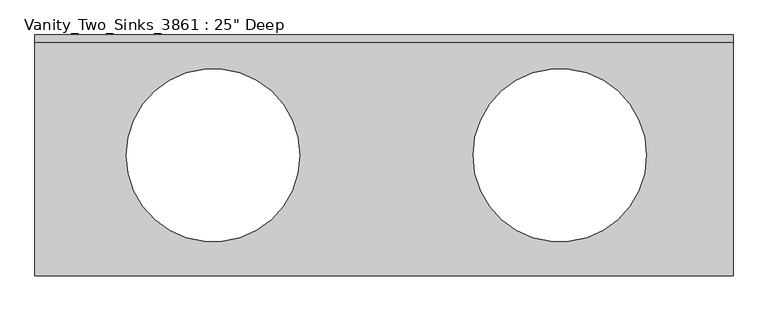
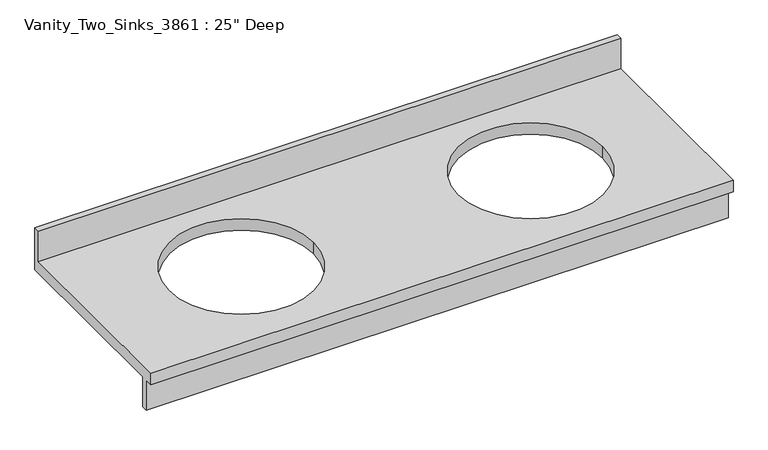
"""IFC4 building model written with IfcOpenShell, lengths in millimetres: furniture geometry."""

import ifcopenshell
import ifcopenshell.guid

model = None  # the IFC model being written
_history = None  # IfcOwnerHistory: only IFC2X3 demands one
_inside = {}  # id of a spatial element -> (the spatial element, [elements in it])
_under = {}  # id of a project, library or spatial element -> (it, [spatial elements below it])
_declared = {}  # id of a project -> (the project, [libraries it declares])
_typed = {}  # id of a type object -> (the type object, [elements of that type])
_made_of = {}  # id of a material, layer set ... -> (it, [elements and type objects made of it])


def new_model(schema):
    """Start an empty IFC model of exactly this schema.

    Asked for "IFC4X3", IfcOpenShell would pick the latest addendum, in which some entities
    have other attributes; the version numbers below select the first issue.
    IFC2X3 requires an IfcOwnerHistory on every rooted entity: one is made here for all.
    """
    global model, _history
    if schema == "IFC4X3":
        model = ifcopenshell.file(schema_version=(4, 3, 0, 0))
    else:
        model = ifcopenshell.file(schema=schema)
    _inside.clear()
    _under.clear()
    _declared.clear()
    _typed.clear()
    _made_of.clear()
    _history = None
    if model.schema == "IFC2X3":
        org = make("IfcOrganization", Name="unknown")
        user = make(
            "IfcPersonAndOrganization",
            ThePerson=make("IfcPerson", FamilyName="unknown"),
            TheOrganization=org,
        )
        app = make(
            "IfcApplication",
            ApplicationDeveloper=org,
            Version="unknown",
            ApplicationFullName="unknown",
            ApplicationIdentifier="unknown",
        )
        _history = make(
            "IfcOwnerHistory",
            OwningUser=user,
            OwningApplication=app,
            ChangeAction="ADDED",
            CreationDate=0,
        )
    return model


def make(cls, **values):
    """One entity of the class cls with the attributes given. An attribute that is None is left unset."""
    return model.create_entity(
        cls, **{name: value for name, value in values.items() if value is not None}
    )


def rooted(cls, **values):
    """An entity with a GlobalId (a new one), such as an element, a storey or a relation."""
    return make(cls, GlobalId=ifcopenshell.guid.new(), OwnerHistory=_history, **values)


def si_unit(unit_type, name, prefix=None):
    """IfcSIUnit, for example si_unit("LENGTHUNIT", "METRE", prefix="MILLI")."""
    return make("IfcSIUnit", UnitType=unit_type, Prefix=prefix, Name=name)


def assignment(units):
    """IfcUnitAssignment: the units of a project."""
    return None if units is None else make("IfcUnitAssignment", Units=units)


def point(xyz):
    """IfcCartesianPoint."""
    return None if xyz is None else make("IfcCartesianPoint", Coordinates=xyz)


def direction(xyz):
    """IfcDirection."""
    return None if xyz is None else make("IfcDirection", DirectionRatios=xyz)


def frame(location, z_axis=None, x_axis=None):
    """IfcAxis2Placement3D, a coordinate frame: its origin and axes. An axis left out is left unset."""
    return make(
        "IfcAxis2Placement3D",
        Location=point(location),
        Axis=direction(z_axis),
        RefDirection=direction(x_axis),
    )


def origin():
    """The frame at (0, 0, 0) with its axes left unset."""
    return frame((0.0, 0.0, 0.0))


def place(relative_to, where):
    """IfcLocalPlacement: puts the frame where relative to a parent placement (None: the world)."""
    return make(
        "IfcLocalPlacement", PlacementRelTo=relative_to, RelativePlacement=where
    )


def context(
    kind, dimensions, precision=None, world=None, true_north=None, identifier=None
):
    """IfcGeometricRepresentationContext, for example the 3D "Model" context."""
    return make(
        "IfcGeometricRepresentationContext",
        ContextIdentifier=identifier,
        ContextType=kind,
        CoordinateSpaceDimension=dimensions,
        Precision=precision,
        WorldCoordinateSystem=world,
        TrueNorth=true_north,
    )


def project(units=None, contexts=None):
    """IfcProject with its units and contexts."""
    return rooted(
        "IfcProject",
        Name="project",
        RepresentationContexts=contexts,
        UnitsInContext=assignment(units),
    )


def spatial(cls, under=None, at=None, **own):
    """A site, building, storey or space (cls), placed at a placement, below another one or the project."""
    s = rooted(cls, ObjectPlacement=at, **own)
    if under is not None:
        _under.setdefault(under.id(), (under, []))[1].append(s)
    return s


def polyline(points):
    """IfcPolyline through the points."""
    return make("IfcPolyline", Points=[point(p) for p in points])


def circle_curve(where, radius):
    """IfcCircle in the frame where."""
    return make("IfcCircle", Position=where, Radius=radius)


def shape(context_of_items, identifier, shape_type, items):
    """IfcShapeRepresentation: the items that make up one representation, for example the "Body"."""
    return make(
        "IfcShapeRepresentation",
        ContextOfItems=context_of_items,
        RepresentationIdentifier=identifier,
        RepresentationType=shape_type,
        Items=items,
    )


def source(mapping_origin, context_of_items, identifier, shape_type, items):
    """IfcRepresentationMap: a shape defined once, which mapped items show again and again."""
    return make(
        "IfcRepresentationMap",
        MappingOrigin=mapping_origin,
        MappedRepresentation=shape(context_of_items, identifier, shape_type, items),
    )


def transform(
    local_origin,
    x_axis=None,
    y_axis=None,
    z_axis=None,
    scale=None,
    scale2=None,
    scale3=None,
    uniform=True,
):
    """IfcCartesianTransformationOperator3D, or its non-uniform kind. x_axis, y_axis, z_axis: its Axis1, 2, 3."""
    if uniform:
        return make(
            "IfcCartesianTransformationOperator3D",
            Axis1=direction(x_axis),
            Axis2=direction(y_axis),
            LocalOrigin=point(local_origin),
            Scale=scale,
            Axis3=direction(z_axis),
        )
    return make(
        "IfcCartesianTransformationOperator3DnonUniform",
        Axis1=direction(x_axis),
        Axis2=direction(y_axis),
        LocalOrigin=point(local_origin),
        Scale=scale,
        Axis3=direction(z_axis),
        Scale2=scale2,
        Scale3=scale3,
    )


def mapped(mapping_source, mapping_target):
    """IfcMappedItem: shows the shape of a source again, moved by a transform."""
    return make(
        "IfcMappedItem", MappingSource=mapping_source, MappingTarget=mapping_target
    )


def made_of(thing, what):
    """Note that an element or type object is made of a material, layer set ...; save() writes the relation."""
    if what is not None:
        _made_of.setdefault(what.id(), (what, []))[1].append(thing)
    return thing


def element(
    cls,
    number,
    at=None,
    inside=None,
    cuts=None,
    type_object=None,
    material=None,
    context=None,
    identifier="Body",
    shape_type=None,
    held_by="IfcProductDefinitionShape",
    body=None,
    shapes=None,
    **own,
):
    """One element of the class cls, such as IfcWall. Its Tag is "e" and its number.

    at: its placement. inside: the storey or other place that contains it. cuts: it is an
    opening in that element (IfcRelVoidsElement). A single representation is given by context,
    identifier, shape_type and body (its items); several are given by shapes. held_by: the class
    of the entity that holds the representations. save() writes the other relations.
    """
    e = rooted(cls, Tag="e%d" % number, ObjectPlacement=at, **own)
    if body is not None:
        shapes = [shape(context, identifier, shape_type, body)]
    if shapes is not None:
        e.Representation = make(held_by, Representations=shapes)
    if inside is not None:
        _inside.setdefault(inside.id(), (inside, []))[1].append(e)
    if cuts is not None:
        rooted(
            "IfcRelVoidsElement", RelatingBuildingElement=cuts, RelatedOpeningElement=e
        )
    if type_object is not None:
        _typed.setdefault(type_object.id(), (type_object, []))[1].append(e)
    return made_of(e, material)


def aggregate(whole, parts):
    """IfcRelAggregates: a whole, such as a stair, and the parts it consists of."""
    return rooted("IfcRelAggregates", RelatingObject=whole, RelatedObjects=parts)


def save(model, path):
    """Write the relations noted so far, then the file.

    IfcRelAggregates (storeys below a building ...), IfcRelContainedInSpatialStructure (elements
    in a storey), IfcRelDefinesByType, IfcRelAssociatesMaterial and IfcRelDeclares: one each for
    every whole, place, type object, material and project.
    """
    for whole, parts in _under.values():
        aggregate(whole, parts)
    for where, things in _inside.values():
        rooted(
            "IfcRelContainedInSpatialStructure",
            RelatedElements=things,
            RelatingStructure=where,
        )
    for kind, things in _typed.values():
        rooted("IfcRelDefinesByType", RelatedObjects=things, RelatingType=kind)
    for what, things in _made_of.values():
        rooted("IfcRelAssociatesMaterial", RelatedObjects=things, RelatingMaterial=what)
    for by, libraries in _declared.values():
        rooted("IfcRelDeclares", RelatingContext=by, RelatedDefinitions=libraries)
    model.write(path)


def plane_surface(at):
    """IfcPlane: the flat surface through the origin of the frame at, square to its z axis."""
    return make("IfcPlane", Position=at)


def revolved_surface(curve, axis_point, axis_direction):
    """IfcSurfaceOfRevolution: the curve turned about the line through axis_point along axis_direction."""
    return make(
        "IfcSurfaceOfRevolution",
        SweptCurve=make("IfcArbitraryOpenProfileDef", ProfileType="CURVE", Curve=curve),
        AxisPosition=make("IfcAxis1Placement", Location=point(axis_point), Axis=direction(axis_direction)),
    )


def advanced_brep(points, edges, surfaces, faces):
    """IfcAdvancedBrep: a solid bounded by faces that lie on surfaces and meet in shared edges.

    An edge is (start, end): straight between two places in points (the first is 0);
    or (start, end, curve); or (start, end, curve, False) where it runs against its curve.
    A face is (place in surfaces, loops), or (place, loops, False) where it looks against
    its surface's normal. A loop lists edges by number (the first is 1), with a minus sign
    where the edge is run from its end to its start. The first loop is the outer one.
    """
    corners = [point(p) for p in points]
    vertices = [make("IfcVertexPoint", VertexGeometry=c) for c in corners]
    made = []
    for start, end, *more in edges:
        made.append(
            make(
                "IfcEdgeCurve",
                EdgeStart=vertices[start],
                EdgeEnd=vertices[end],
                EdgeGeometry=more[0] if more else make("IfcPolyline", Points=[corners[start], corners[end]]),
                SameSense=more[1] if len(more) > 1 else True,
            )
        )
    hull = []
    for where, loops, *sense in faces:
        bounds = []
        for j, loop in enumerate(loops):
            ring = [make("IfcOrientedEdge", EdgeElement=made[abs(k) - 1], Orientation=k > 0) for k in loop]
            bounds.append(
                make(
                    "IfcFaceOuterBound" if j == 0 else "IfcFaceBound",
                    Bound=make("IfcEdgeLoop", EdgeList=ring),
                    Orientation=True,
                )
            )
        hull.append(make("IfcAdvancedFace", Bounds=bounds, FaceSurface=surfaces[where], SameSense=sense[0] if sense else True))
    return make("IfcAdvancedBrep", Outer=make("IfcClosedShell", CfsFaces=hull))


def furniture_801237fe(model_context):
    return source(origin(), model_context, "Body", "AdvancedBrep", [
        advanced_brep(
        [(-1327.4622951, -635.0, 863.6), (514.0377049, -635.0, 863.6), (514.0377049, -19.05, 863.6), (-1327.4622951, -19.05, 863.6), (285.4377049, -317.5, 863.6), (-171.7622951, -317.5, 863.6), (-628.9622951, -317.5, 863.6), (-1086.1622951, -317.5, 863.6), (514.0377049, -635.0, 825.5), (-1327.4622951, -635.0, 825.5), (-1327.4622951, -609.6, 825.5), (514.0377049, -609.6, 825.5), (-1327.4622951, 0.0, 825.5), (514.0377049, 0.0, 825.5), (514.0377049, -590.55, 825.5), (-1327.4622951, -590.55, 825.5), (-171.7622951, -317.5, 825.5), (285.4377049, -317.5, 825.5), (-1086.1622951, -317.5, 825.5), (-628.9622951, -317.5, 825.5), (-1327.4622951, 0.0, 965.2), (514.0377049, 0.0, 965.2), (-1327.4622951, -19.05, 965.2), (-1327.4622951, -590.55, 723.9), (-1327.4622951, -609.6, 723.9), (514.0377049, -609.6, 723.9), (514.0377049, -590.55, 723.9), (514.0377049, -19.05, 965.2)],
        [
            (0, 1),
            (1, 2),
            (2, 3),
            (3, 0),
            (4, 5, circle_curve(frame((56.8377049, -317.5, 863.6), z_axis=(0.0, 0.0, -1.0), x_axis=(1.0, 0.0, 0.0)), 228.6)),
            (5, 4, circle_curve(frame((56.8377049, -317.5, 863.6), z_axis=(0.0, 0.0, -1.0), x_axis=(1.0, 0.0, 0.0)), 228.6)),
            (6, 7, circle_curve(frame((-857.5622951, -317.5, 863.6), z_axis=(0.0, 0.0, -1.0), x_axis=(1.0, 0.0, 0.0)), 228.6)),
            (7, 6, circle_curve(frame((-857.5622951, -317.5, 863.6), z_axis=(0.0, 0.0, -1.0), x_axis=(1.0, 0.0, 0.0)), 228.6)),
            (8, 9),
            (9, 10),
            (10, 11),
            (11, 8),
            (12, 13),
            (13, 14),
            (14, 15),
            (15, 12),
            (16, 17, circle_curve(frame((56.8377049, -317.5, 825.5), z_axis=(0.0, 0.0, 1.0), x_axis=(1.0, 0.0, 0.0)), 228.6)),
            (17, 16, circle_curve(frame((56.8377049, -317.5, 825.5), z_axis=(0.0, 0.0, 1.0), x_axis=(1.0, 0.0, 0.0)), 228.6)),
            (18, 19, circle_curve(frame((-857.5622951, -317.5, 825.5), z_axis=(0.0, 0.0, 1.0), x_axis=(1.0, 0.0, 0.0)), 228.6)),
            (19, 18, circle_curve(frame((-857.5622951, -317.5, 825.5), z_axis=(0.0, 0.0, 1.0), x_axis=(1.0, 0.0, 0.0)), 228.6)),
            (12, 20),
            (20, 21),
            (21, 13),
            (9, 0),
            (3, 22),
            (22, 20),
            (15, 23),
            (23, 24),
            (24, 10),
            (8, 1),
            (11, 25),
            (25, 26),
            (26, 14),
            (21, 27),
            (27, 2),
            (4, 17),
            (16, 5),
            (22, 27),
            (6, 19),
            (18, 7),
            (25, 24),
            (23, 26),
        ],
        [
            plane_surface(frame((-1327.4622951, 0.0, 863.6), z_axis=(0.0, 0.0, 1.0), x_axis=(-1.0, 0.0, 0.0))),
            plane_surface(frame((-1327.4622951, 0.0, 825.5), z_axis=(0.0, 0.0, -1.0), x_axis=(1.0, 0.0, 0.0))),
            plane_surface(frame((514.0377049, 0.0, 863.6), z_axis=(0.0, 1.0, 0.0), x_axis=(0.0, 0.0, -1.0))),
            plane_surface(frame((-1327.4622951, 0.0, 863.6), z_axis=(-1.0, 0.0, 0.0), x_axis=(0.0, 0.0, -1.0))),
            plane_surface(frame((-1327.4622951, -635.0, 863.6), z_axis=(0.0, -1.0, 0.0), x_axis=(0.0, 0.0, -1.0))),
            plane_surface(frame((514.0377049, -635.0, 863.6), z_axis=(1.0, 0.0, 0.0), x_axis=(0.0, 0.0, -1.0))),
            revolved_surface(polyline([(285.43770489999997, -317.5, 863.6), (285.43770489999997, -317.5, 825.5)]), (56.8377049, -317.5, 825.5), (0.0, 0.0, 1.0)),
            plane_surface(frame((-1327.4622951, 0.0, 965.2), z_axis=(0.0, 0.0, 1.0), x_axis=(0.0, -1.0, 0.0))),
            plane_surface(frame((-1327.4622951, -19.05, 965.2), z_axis=(0.0, -1.0, 0.0), x_axis=(0.0, 0.0, -1.0))),
            revolved_surface(polyline([(-628.9622951, -317.5, 863.6), (-628.9622951, -317.5, 825.5)]), (-857.5622951, -317.5, 825.5), (0.0, 0.0, 1.0)),
            plane_surface(frame((-1327.4622951, -590.55, 723.9), z_axis=(0.0, 0.0, -1.0), x_axis=(1.0, 0.0, 0.0))),
            plane_surface(frame((514.0377049, -590.55, 825.5), z_axis=(0.0, 1.0, 0.0), x_axis=(0.0, 0.0, -1.0))),
            plane_surface(frame((-1327.4622951, -609.6, 825.5), z_axis=(0.0, -1.0, 0.0), x_axis=(0.0, 0.0, -1.0))),
        ],
        [
            (0, [[1, 2, 3, 4], [5, 6], [7, 8]]),
            (1, [[9, 10, 11, 12]]),
            (1, [[13, 14, 15, 16], [17, 18], [19, 20]]),
            (2, [[-13, 21, 22, 23]]),
            (3, [[24, -4, 25, 26, -21, -16, 27, 28, 29, -10]]),
            (4, [[-1, -24, -9, 30]]),
            (5, [[-30, -12, 31, 32, 33, -14, -23, 34, 35, -2]]),
            (6, [[36, -17, 37, -5]]),
            (6, [[-36, -6, -37, -18]]),
            (7, [[-26, 38, -34, -22]]),
            (8, [[-38, -25, -3, -35]]),
            (9, [[39, -19, 40, -7]]),
            (9, [[-39, -8, -40, -20]]),
            (10, [[-32, 41, -28, 42]]),
            (11, [[-42, -27, -15, -33]]),
            (12, [[-41, -31, -11, -29]]),
        ],
    ),
    ])


if __name__ == "__main__":
    model = new_model("IFC4")
    model_context = context("Model", 3, world=origin())
    ifc_project = project(units=[si_unit("LENGTHUNIT", "METRE", prefix="MILLI")], contexts=[model_context])
    site = spatial("IfcSite", under=ifc_project)
    building = spatial("IfcBuilding", under=site)
    placement = place(None, origin())
    furniture_shape = furniture_801237fe(model_context)
    element("IfcFurniture", 1, ObjectType="Vanity_Two_Sinks_3861 : 25\" Deep", at=placement, inside=building, context=model_context, shape_type="MappedRepresentation", body=[
        mapped(furniture_shape, transform((0.0, 0.0, 0.0), x_axis=(1.0, 0.0, 0.0), y_axis=(0.0, 1.0, 0.0), z_axis=(0.0, 0.0, 1.0))),
    ])
    save(model, "model.ifc")

# Revit data of these elements
# Type "Vanity_Two_Sinks_3861 : 25\" Deep"
#   Assembly Code = "C1030400"
#   Sink Location Right [instance default] = 1' - 6"
#   Counter Thickness = 0' - 1 1/2"
#   Depth = 2' - 1"
#   Height = 2' - 10"
#   Length [instance default] = 6' - 0"
#   Sink Location Left [instance default] = 1' - 6"
#   Sink to Back Wall = 0' - 4"
#   Sink Opening Width [instance default] = 1' - 5"
#   Counter Top = Casework - Vanity Top
#   Width = 0
# Element 1 (IfcFurniture, "Vanity_Two_Sinks_3861 : 25\" Deep")
#   Length = 6' - 0 1/2"
#   Sink Location Left = 1' - 6 1/2"
#   Materials on its faces: "Casework - Vanity Top"
# Materials
#   "Casework - Vanity Top": class "Unassigned", colour RGB 210 200 171, transparency 0, Comments = "Rendering appearance not upgraded "
